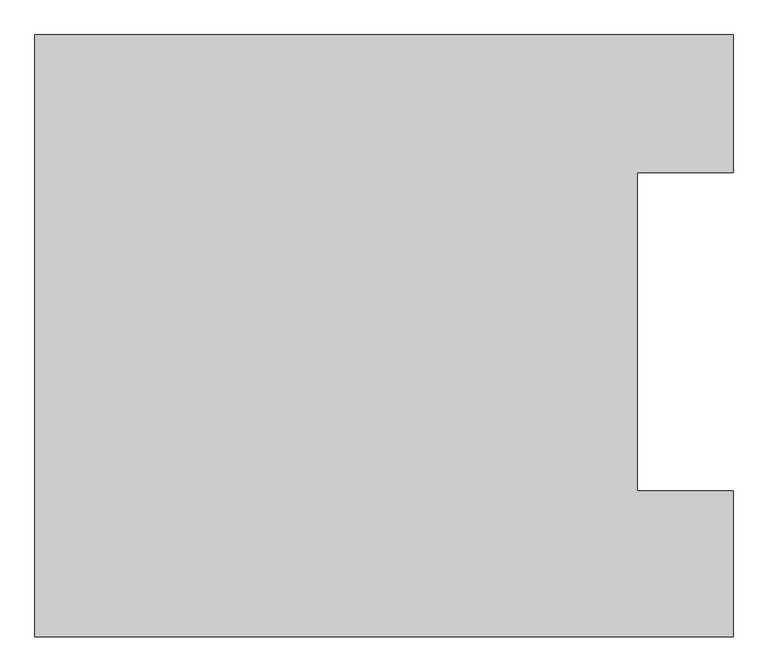
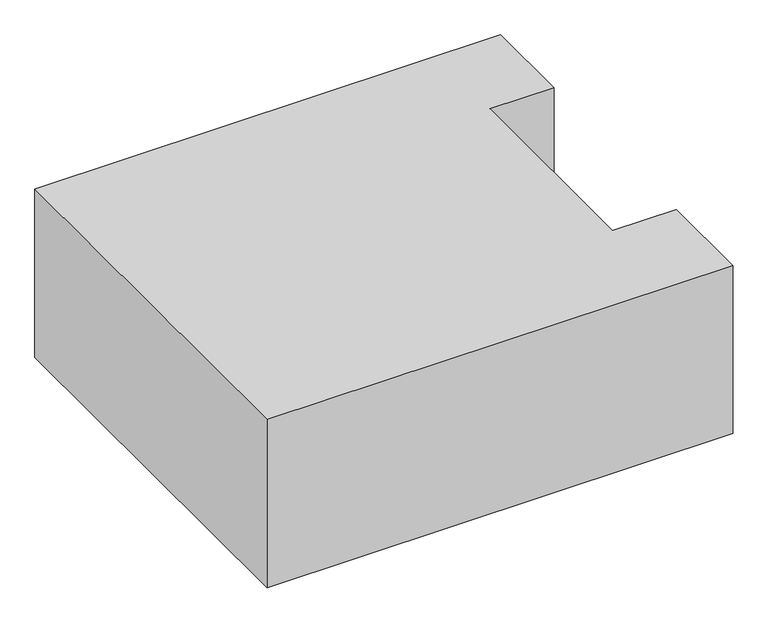
"""IFC4 building model written with IfcOpenShell, lengths in millimetres: proxy geometry, 0_3d."""

from ifc_helpers import new_model, si_unit, origin, origin_with_axes, place, context, project, spatial, polyline, outline, extrude, source, transform, mapped, element, save


def generic_models_2dafeef2(model_context):
    return source(origin(), model_context, "Body", "SweptSolid", [
        extrude(outline(polyline([(6550.0, 0.0), (0.0, 0.0), (0.0, 5650.0), (6550.0, 5650.0), (6550.0, 4357.8), (5650.0, 4357.8), (5650.0, 1367.8), (6550.0, 1367.8), (6550.0, 0.0)])), origin_with_axes(), (0.0, 0.0, 1.0), 2500.0),
    ])


if __name__ == "__main__":
    model = new_model("IFC4")
    model_context = context("Model", 3, world=origin())
    ifc_project = project(units=[si_unit("LENGTHUNIT", "METRE", prefix="MILLI")], contexts=[model_context])
    site = spatial("IfcSite", under=ifc_project)
    building = spatial("IfcBuilding", under=site)
    placement = place(None, origin())
    generic_models_shape = generic_models_2dafeef2(model_context)
    element("IfcBuildingElementProxy", 1, Name="0_3d", ObjectType="0_3d", at=placement, inside=building, context=model_context, shape_type="MappedRepresentation", body=[
        mapped(generic_models_shape, transform((0.0, 0.0, 0.0), x_axis=(1.0, 0.0, 0.0), y_axis=(0.0, 1.0, 0.0), z_axis=(0.0, 0.0, 1.0))),
    ])
    save(model, "model.ifc")

# Revit data of these elements
# Element 1 (IfcBuildingElementProxy, "0_3d")
#   Materials on its faces: "*1"
# Materials
#   "*1": class "Unassigned", colour RGB 175 175 175, transparency 0
